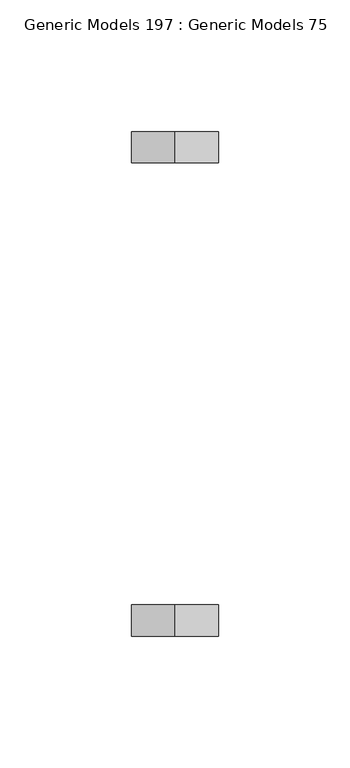
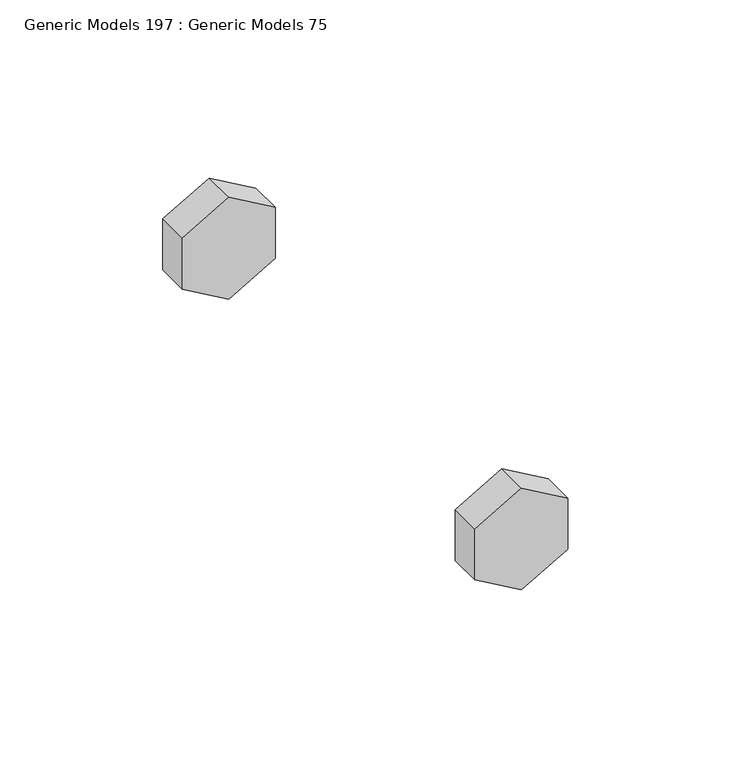
"""IFC4 building model written with IfcOpenShell, lengths in millimetres: proxy geometry, Generic Models 197 : Generic Models 75."""

from ifc_helpers import new_model, si_unit, frame, origin, place, context, project, spatial, polyline, outline, extrude, source, transform, mapped, element, save


def generic_models_197_generic_models_75_92a70932(model_context):
    return source(origin(), model_context, "Body", "SweptSolid", [
        extrude(outline(polyline([(271833.975, 31991.9073871), (271853.025, 31991.9073871), (271862.55, 31975.4096032), (271853.025, 31958.9118192), (271833.975, 31958.9118192), (271824.45, 31975.4096032), (271833.975, 31991.9073871)])), frame((0.0, 35193.7770442, 0.0), z_axis=(0.0, 1.0, 0.0), x_axis=(0.0, 0.0, 1.0)), (0.0, 0.0, 1.0), 11.90625),
        extrude(outline(polyline([(271833.975, 31991.9073871), (271853.025, 31991.9073871), (271862.55, 31975.4096032), (271853.025, 31958.9118192), (271833.975, 31958.9118192), (271824.45, 31975.4096032), (271833.975, 31991.9073871)])), frame((0.0, 35373.5614192, 0.0), z_axis=(0.0, 1.0, 0.0), x_axis=(0.0, 0.0, 1.0)), (0.0, 0.0, 1.0), 11.90625),
    ])


if __name__ == "__main__":
    model = new_model("IFC4")
    model_context = context("Model", 3, world=origin())
    ifc_project = project(units=[si_unit("LENGTHUNIT", "METRE", prefix="MILLI")], contexts=[model_context])
    site = spatial("IfcSite", under=ifc_project)
    building = spatial("IfcBuilding", under=site)
    placement = place(None, origin())
    generic_models_197_generic_models_75_shape = generic_models_197_generic_models_75_92a70932(model_context)
    element("IfcBuildingElementProxy", 1, Name="Generic Models 197 : Generic Models 75", ObjectType="Generic Models 197 : Generic Models 75", at=placement, inside=building, context=model_context, shape_type="MappedRepresentation", body=[
        mapped(generic_models_197_generic_models_75_shape, transform((0.0, 0.0, 0.0), x_axis=(1.0, 0.0, 0.0), y_axis=(0.0, 1.0, 0.0), z_axis=(0.0, 0.0, 1.0))),
    ])
    save(model, "model.ifc")
